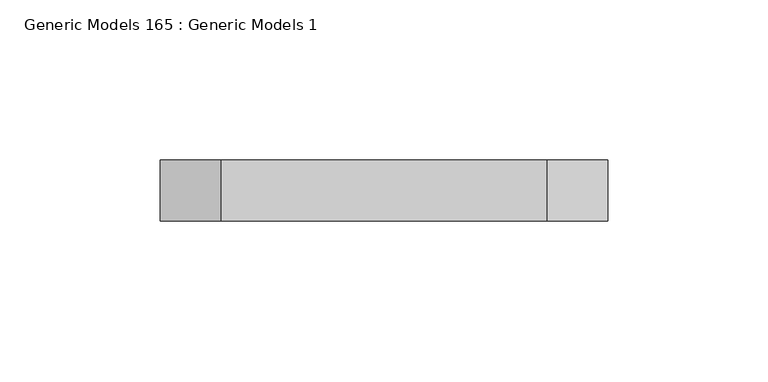
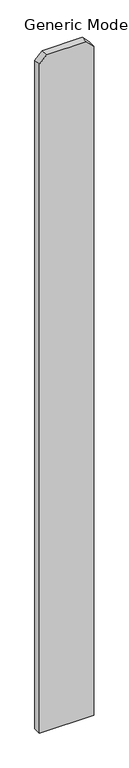
"""IFC4 building model written with IfcOpenShell, lengths in millimetres: proxy geometry, Generic Models 165 : Generic Models 1."""

from ifc_helpers import new_model, si_unit, frame, origin, place, context, project, spatial, polyline, outline, extrude, source, transform, mapped, element, save


def generic_models_165_generic_models_1_5258939b(model_context):
    return source(origin(), model_context, "Body", "SweptSolid", [
        extrude(outline(polyline([(76.2, -249658.1875), (1885.95, -249658.1875), (1905.0, -249677.2375), (1905.0, -249778.8375), (1885.95, -249797.8875), (76.2, -249797.8875), (76.2, -249658.1875)])), frame((0.0, 547.6875, 0.0), z_axis=(0.0, 1.0, 0.0), x_axis=(0.0, 0.0, 1.0)), (0.0, 0.0, 1.0), 19.05),
    ])


if __name__ == "__main__":
    model = new_model("IFC4")
    model_context = context("Model", 3, world=origin())
    ifc_project = project(units=[si_unit("LENGTHUNIT", "METRE", prefix="MILLI")], contexts=[model_context])
    site = spatial("IfcSite", under=ifc_project)
    building = spatial("IfcBuilding", under=site)
    placement = place(None, origin())
    generic_models_165_generic_models_1_shape = generic_models_165_generic_models_1_5258939b(model_context)
    element("IfcBuildingElementProxy", 1, Name="Generic Models 165 : Generic Models 1", ObjectType="Generic Models 165 : Generic Models 1", at=placement, inside=building, context=model_context, shape_type="MappedRepresentation", body=[
        mapped(generic_models_165_generic_models_1_shape, transform((0.0, 0.0, 0.0), x_axis=(1.0, 0.0, 0.0), y_axis=(0.0, 1.0, 0.0), z_axis=(0.0, 0.0, 1.0))),
    ])
    save(model, "model.ifc")

# Revit data of these elements
# Element 1 (IfcBuildingElementProxy, "Generic Models 165 : Generic Models 1")
#   Materials on its faces: "VERTICAL 1X6 CEDAR PLANKS W/ CLEAR WOOD SEALER"
# Materials
#   "VERTICAL 1X6 CEDAR PLANKS W/ CLEAR WOOD SEALER": class "Wood", colour RGB 234 198 147, transparency 0, Description = "Pinus Echinata", Cost = 0
